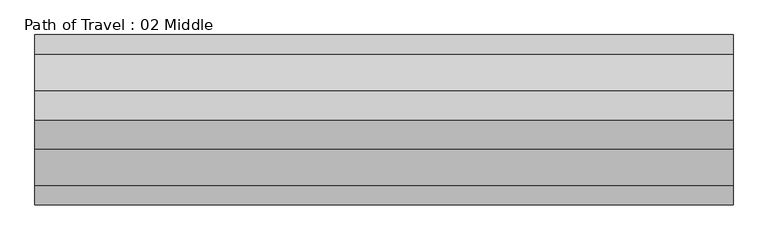
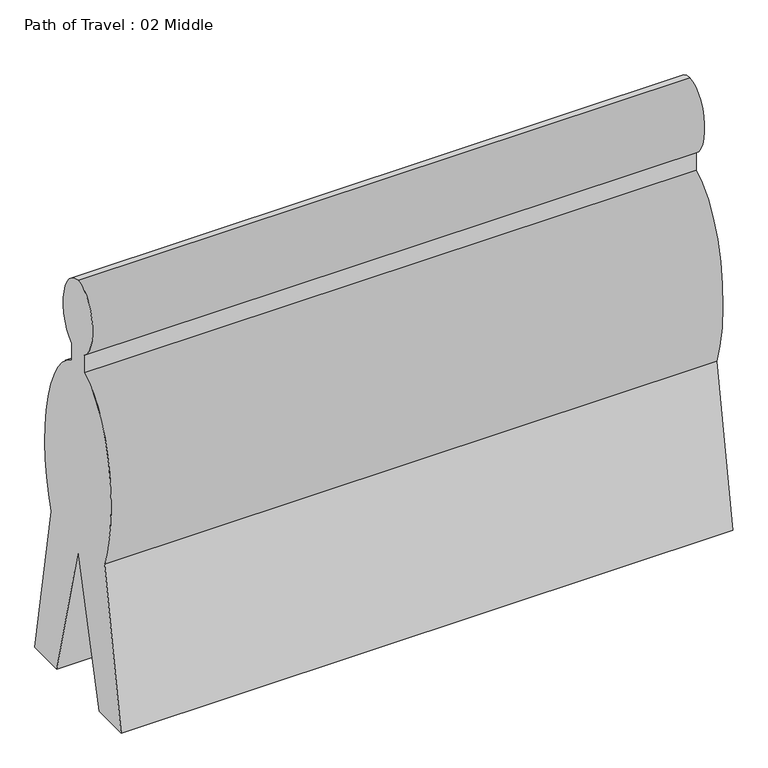
"""IFC4 building model written with IfcOpenShell, lengths in millimetres: proxy geometry, Path of Travel : 02 Middle."""

from ifc_helpers import new_model, si_unit, point, frame, origin, place, context, project, spatial, ellipse_curve, trimmed, source, transform, mapped, element, save
from ifc_brep_helpers import plane_surface, extruded_surface, advanced_brep


def path_of_travel_02_middle_d41fa50e(model_context):
    return source(origin(), model_context, "Body", "AdvancedBrep", [
        advanced_brep(
        [(227.5554837, 0.0, 1727.2), (227.5554837, 42.9018657, 1436.6534209), (227.5554837, 42.9018657, 1363.4763406), (227.5554837, 184.1186263, 643.4144547), (227.5554837, 297.5699544, 0.0), (227.5554837, 145.6574193, 0.0), (227.5554837, 0.0, 584.2), (227.5554837, -145.6574193, 0.0), (227.5554837, -297.5699544, 0.0), (227.5554837, -184.1186263, 643.4144547), (227.5554837, -42.9018657, 1363.4763406), (227.5554837, -42.9018657, 1436.6534209), (2665.9554837, 0.0, 1727.2), (2665.9554837, -42.9018657, 1436.6534209), (2665.9554837, -42.9018657, 1363.4763406), (2665.9554837, -184.1186263, 643.4144547), (2665.9554837, -297.5699544, 0.0), (2665.9554837, -145.6574193, 0.0), (2665.9554837, 0.0, 584.2), (2665.9554837, 145.6574193, 0.0), (2665.9554837, 297.5699544, 0.0), (2665.9554837, 184.1186263, 643.4144547), (2665.9554837, 42.9018657, 1363.4763406), (2665.9554837, 42.9018657, 1436.6534209)],
        [
            (0, 1, ellipse_curve(frame((227.5554837, 0.0, 1574.8), z_axis=(-1.0, 0.0, 0.0), x_axis=(0.0, 0.0, 1.0)), 152.4, 101.6)),
            (1, 2),
            (2, 3, ellipse_curve(frame((227.5554837, 0.0, 914.4), z_axis=(-1.0, 0.0, 0.0), x_axis=(0.0, 0.0, -1.0)), 457.2, 228.6)),
            (3, 4),
            (4, 5),
            (5, 6),
            (6, 7),
            (7, 8),
            (8, 9),
            (9, 10, ellipse_curve(frame((227.5554837, 0.0, 914.4), z_axis=(-1.0, 0.0, 0.0), x_axis=(0.0, 0.0, -1.0)), 457.2, 228.6)),
            (10, 11),
            (11, 0, ellipse_curve(frame((227.5554837, 0.0, 1574.8), z_axis=(-1.0, 0.0, 0.0), x_axis=(0.0, 0.0, 1.0)), 152.4, 101.6)),
            (12, 13, ellipse_curve(frame((2665.9554837, 0.0, 1574.8), z_axis=(1.0, 0.0, 0.0), x_axis=(0.0, 0.0, 1.0)), 152.4, 101.6)),
            (13, 14),
            (14, 15, ellipse_curve(frame((2665.9554837, 0.0, 914.4), z_axis=(1.0, 0.0, 0.0), x_axis=(0.0, 0.0, -1.0)), 457.2, 228.6)),
            (15, 16),
            (16, 17),
            (17, 18),
            (18, 19),
            (19, 20),
            (20, 21),
            (21, 22, ellipse_curve(frame((2665.9554837, 0.0, 914.4), z_axis=(1.0, 0.0, 0.0), x_axis=(0.0, 0.0, -1.0)), 457.2, 228.6)),
            (22, 23),
            (23, 12, ellipse_curve(frame((2665.9554837, 0.0, 1574.8), z_axis=(1.0, 0.0, 0.0), x_axis=(0.0, 0.0, 1.0)), 152.4, 101.6)),
            (0, 12),
            (23, 1),
            (22, 2),
            (21, 3),
            (20, 4),
            (19, 5),
            (18, 6),
            (17, 7),
            (16, 8),
            (15, 9),
            (14, 10),
            (13, 11),
        ],
        [
            plane_surface(frame((227.5554837, 0.0, 0.0), z_axis=(-1.0, 0.0, 0.0), x_axis=(0.0, 0.0, 1.0))),
            plane_surface(frame((2665.9554837, 0.0, 0.0), z_axis=(1.0, 0.0, 0.0), x_axis=(0.0, 0.0, 1.0))),
            extruded_surface(trimmed(ellipse_curve(frame((2665.9554837, 0.0, 1574.8), z_axis=(-1.0, 0.0, 0.0), x_axis=(0.0, 0.0, 1.0)), 152.4, 101.6), [point((2665.9554837, 0.0, 1727.2))], [point((2665.9554837, 42.9018657, 1436.6534209))], True, "CARTESIAN"), (-2438.4, 0.0, 0.0), 2438.4),
            plane_surface(frame((227.5554837, 42.9018657, 1436.6534209), z_axis=(0.0, 1.0, 0.0), x_axis=(1.0, 0.0, 0.0))),
            extruded_surface(trimmed(ellipse_curve(frame((2665.9554837, 0.0, 914.4), z_axis=(-1.0, 0.0, 0.0), x_axis=(0.0, 0.0, -1.0)), 457.2, 228.6), [point((2665.9554837, 42.9018657, 1363.4763406))], [point((2665.9554837, 184.1186263, 643.4144547))], True, "CARTESIAN"), (-2438.4, 0.0, 0.0), 2438.4),
            plane_surface(frame((227.5554837, 184.1186263, 643.4144547), z_axis=(0.0, 0.9848077530122078, 0.17364817766693205), x_axis=(1.0, 0.0, 0.0))),
            plane_surface(frame((227.5554837, 297.5699544, 0.0), z_axis=(0.0, 0.0, -1.0), x_axis=(1.0, 0.0, 0.0))),
            plane_surface(frame((227.5554837, 145.6574193, 0.0), z_axis=(0.0, -0.9702957262760199, -0.2419218955995739), x_axis=(1.0, 0.0, 0.0))),
            plane_surface(frame((227.5554837, 0.0, 584.2), z_axis=(0.0, 0.9702957262759961, -0.24192189559966923), x_axis=(1.0, 0.0, 0.0))),
            plane_surface(frame((227.5554837, -145.6574193, 0.0), z_axis=(0.0, 0.0, -1.0), x_axis=(1.0, 0.0, 0.0))),
            plane_surface(frame((227.5554837, -297.5699544, 0.0), z_axis=(0.0, -0.984807753012208, 0.17364817766693066), x_axis=(1.0, 0.0, 0.0))),
            extruded_surface(trimmed(ellipse_curve(frame((2665.9554837, 0.0, 914.4), z_axis=(-1.0, 0.0, 0.0), x_axis=(0.0, 0.0, -1.0)), 457.2, 228.6), [point((2665.9554837, -184.1186263, 643.4144547))], [point((2665.9554837, -42.9018657, 1363.4763406))], True, "CARTESIAN"), (-2438.4, 0.0, 0.0), 2438.4),
            plane_surface(frame((227.5554837, -42.9018657, 1363.4763406), z_axis=(0.0, -1.0, 0.0), x_axis=(1.0, 0.0, 0.0))),
            extruded_surface(trimmed(ellipse_curve(frame((2665.9554837, 0.0, 1574.8), z_axis=(-1.0, 0.0, 0.0), x_axis=(0.0, 0.0, 1.0)), 152.4, 101.6), [point((2665.9554837, -42.9018657, 1436.6534209))], [point((2665.9554837, 0.0, 1727.2))], True, "CARTESIAN"), (-2438.4, 0.0, 0.0), 2438.4),
        ],
        [
            (0, [[1, 2, 3, 4, 5, 6, 7, 8, 9, 10, 11, 12]]),
            (1, [[13, 14, 15, 16, 17, 18, 19, 20, 21, 22, 23, 24]]),
            (2, [[-1, 25, -24, 26]]),
            (3, [[-2, -26, -23, 27]]),
            (4, [[-3, -27, -22, 28]]),
            (5, [[-4, -28, -21, 29]]),
            (6, [[-5, -29, -20, 30]]),
            (7, [[-6, -30, -19, 31]]),
            (8, [[-7, -31, -18, 32]]),
            (9, [[-8, -32, -17, 33]]),
            (10, [[-9, -33, -16, 34]]),
            (11, [[-10, -34, -15, 35]]),
            (12, [[-11, -35, -14, 36]]),
            (13, [[-12, -36, -13, -25]]),
        ],
    ),
    ])


if __name__ == "__main__":
    model = new_model("IFC4")
    model_context = context("Model", 3, world=origin())
    ifc_project = project(units=[si_unit("LENGTHUNIT", "METRE", prefix="MILLI")], contexts=[model_context])
    site = spatial("IfcSite", under=ifc_project)
    building = spatial("IfcBuilding", under=site)
    placement = place(None, origin())
    path_of_travel_02_middle_shape = path_of_travel_02_middle_d41fa50e(model_context)
    element("IfcBuildingElementProxy", 1, Name="Path of Travel : 02 Middle", ObjectType="Path of Travel : 02 Middle", at=placement, inside=building, context=model_context, shape_type="MappedRepresentation", body=[
        mapped(path_of_travel_02_middle_shape, transform((0.0, 0.0, 0.0), x_axis=(1.0, 0.0, 0.0), y_axis=(0.0, 1.0, 0.0), z_axis=(0.0, 0.0, 1.0))),
    ])
    save(model, "model.ifc")

# Revit data of these elements
# Type "Path of Travel : 02 Middle"
#   Path of Egress [instance default] = 4' - 0"
#   built-in parameter 1001306 [instance default] = 4 (stored number, unit not read)
#   Dot at Start = no
#   Arrow in Middle = yes
#   Arrow at End = no
#   Egress Path = none
# Element 1 (IfcBuildingElementProxy, "Path of Travel : 02 Middle")
#   Path of Egress = 8' - 0"
#   built-in parameter 1001306 = 8 (stored number, unit not read)
#   Materials on its faces: "Egress Path Solid"
# Materials
#   "Egress Path Solid": class "Unassigned", colour RGB 255 128 64, transparency 0.75, Comments = "Rendering appearance not upgraded "
